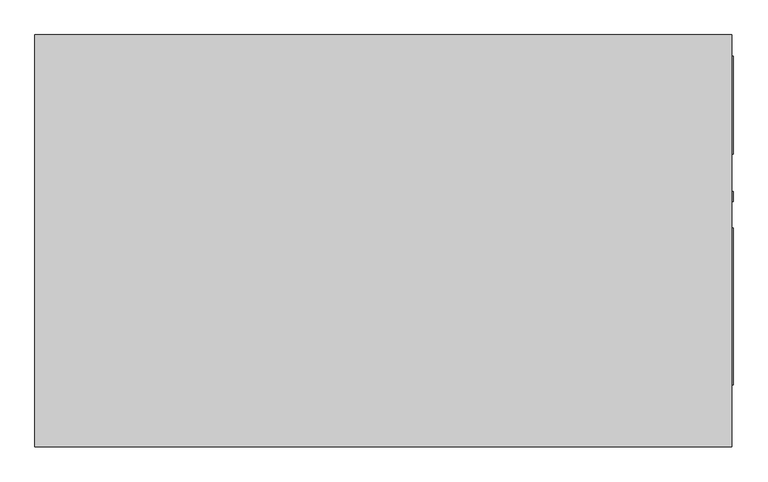
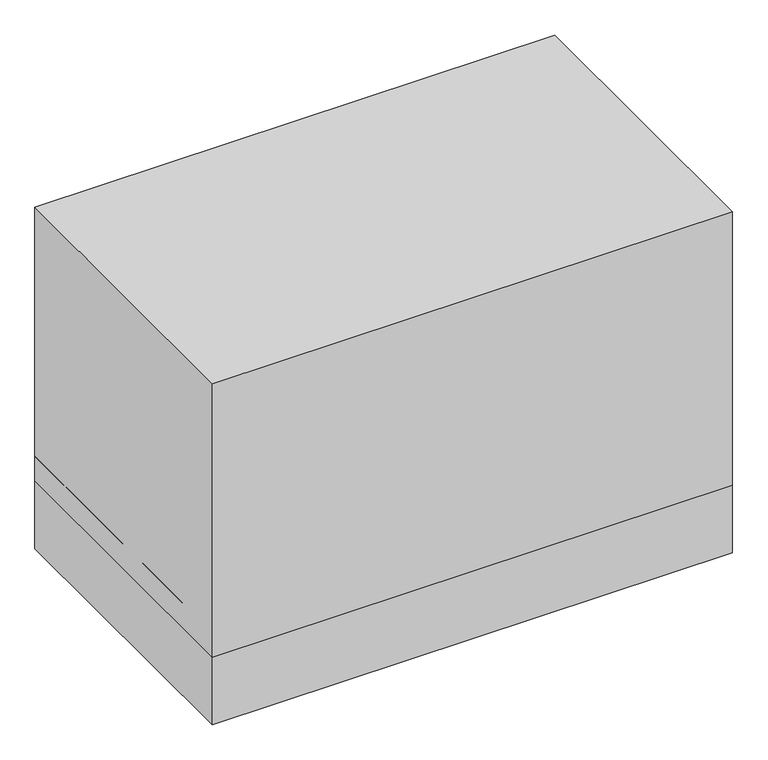
"""IFC4 building model written with IfcOpenShell, lengths in millimetres: proxy geometry, Carrier_48TC_Standard_Efficiency_Gas_Heat_Electric_Cooling_Packaged_Rooftop_Unit_3_to_15_nominal_tons : 6 ton 48TC**07."""

from ifc_helpers import new_model, si_unit, point, frame, frame_2d, origin, origin_with_axes, place, context, project, spatial, polyline, circle_curve, trimmed, segment, composite_curve, outline, extrude, source, transform, mapped, element, save
from ifc_brep_helpers import plane_surface, revolved_surface, advanced_brep


def mechanical_equipment_a9af85ce(model_context):
    return source(origin(), model_context, "Body", "SolidModel", [
        extrude(outline(composite_curve([segment(trimmed(circle_curve(frame_2d((120.65, 438.15)), 13.2953125), [point((107.3546875, 438.15))], [point((133.9453125, 438.15))], False, "CARTESIAN"), True, "CONTINUOUS"), segment(trimmed(circle_curve(frame_2d((120.65, 438.15)), 13.2953125), [point((133.9453125, 438.15))], [point((107.3546875, 438.15))], False, "CARTESIAN"), True, "CONTINUOUS")], self_intersect=False)), frame((944.5625, 0.0, 0.0), z_axis=(1.0, 0.0, 0.0), x_axis=(0.0, 1.0, 0.0)), (0.0, 0.0, 1.0), 3.175),
        advanced_brep(
        [(944.5625, 558.8, 1311.275), (-944.5625, 558.8, 1311.275), (-944.5625, -558.8, 1311.275), (944.5625, -558.8, 1311.275), (944.5625, 558.8, 260.35), (944.5625, -558.8, 260.35), (-944.5625, -558.8, 260.35), (-944.5625, 558.8, 260.35), (858.8375, -400.05, 260.35), (858.8375, 0.0, 260.35), (550.8625, 0.0, 260.35), (550.8625, -400.05, 260.35), (858.8375, 463.55, 260.35), (207.9625, 463.55, 260.35), (207.9625, 187.325, 260.35), (858.8375, 187.325, 260.35), (284.7578125, -88.9, 260.35), (258.1671875, -88.9, 260.35), (-298.45, -247.65, 260.35), (-320.675, -247.65, 260.35), (-295.275, -149.225, 260.35), (-323.85, -149.225, 260.35), (-294.48125, -98.425, 260.35), (-324.64375, -98.425, 260.35), (858.8375, -400.05, 381.0), (550.8625, -400.05, 381.0), (550.8625, 0.0, 381.0), (858.8375, 0.0, 381.0), (858.8375, 463.55, 381.0), (858.8375, 187.325, 381.0), (207.9625, 187.325, 381.0), (207.9625, 463.55, 381.0), (284.7578125, -88.9, 415.925), (258.1671875, -88.9, 415.925), (-298.45, -247.65, 415.925), (-320.675, -247.65, 415.925), (-295.275, -149.225, 415.925), (-323.85, -149.225, 415.925), (-294.48125, -98.425, 415.925), (-324.64375, -98.425, 415.925)],
        [
            (0, 1),
            (1, 2),
            (2, 3),
            (3, 0),
            (4, 5),
            (5, 6),
            (6, 7),
            (7, 4),
            (8, 9),
            (9, 10),
            (10, 11),
            (11, 8),
            (12, 13),
            (13, 14),
            (14, 15),
            (15, 12),
            (16, 17, circle_curve(frame((271.4625, -88.9, 260.35), z_axis=(0.0, 0.0, 1.0), x_axis=(-1.0, 0.0, 0.0)), 13.2953125)),
            (17, 16, circle_curve(frame((271.4625, -88.9, 260.35), z_axis=(0.0, 0.0, 1.0), x_axis=(-1.0, 0.0, 0.0)), 13.2953125)),
            (18, 19, circle_curve(frame((-309.5625, -247.65, 260.35), z_axis=(0.0, 0.0, 1.0), x_axis=(-1.0, 0.0, 0.0)), 11.1125)),
            (19, 18, circle_curve(frame((-309.5625, -247.65, 260.35), z_axis=(0.0, 0.0, 1.0), x_axis=(-1.0, 0.0, 0.0)), 11.1125)),
            (20, 21, circle_curve(frame((-309.5625, -149.225, 260.35), z_axis=(0.0, 0.0, 1.0), x_axis=(-1.0, 0.0, 0.0)), 14.2875)),
            (21, 20, circle_curve(frame((-309.5625, -149.225, 260.35), z_axis=(0.0, 0.0, 1.0), x_axis=(-1.0, 0.0, 0.0)), 14.2875)),
            (22, 23, circle_curve(frame((-309.5625, -98.425, 260.35), z_axis=(0.0, 0.0, 1.0), x_axis=(-1.0, 0.0, 0.0)), 15.08125)),
            (23, 22, circle_curve(frame((-309.5625, -98.425, 260.35), z_axis=(0.0, 0.0, 1.0), x_axis=(-1.0, 0.0, 0.0)), 15.08125)),
            (0, 4),
            (7, 1),
            (6, 2),
            (5, 3),
            (24, 25),
            (25, 26),
            (26, 27),
            (27, 24),
            (27, 9),
            (8, 24),
            (26, 10),
            (25, 11),
            (28, 29),
            (29, 30),
            (30, 31),
            (31, 28),
            (31, 13),
            (12, 28),
            (30, 14),
            (29, 15),
            (32, 33, circle_curve(frame((271.4625, -88.9, 415.925), z_axis=(0.0, 0.0, -1.0), x_axis=(-1.0, 0.0, 0.0)), 13.2953125)),
            (33, 32, circle_curve(frame((271.4625, -88.9, 415.925), z_axis=(0.0, 0.0, -1.0), x_axis=(-1.0, 0.0, 0.0)), 13.2953125)),
            (33, 17),
            (16, 32),
            (34, 35, circle_curve(frame((-309.5625, -247.65, 415.925), z_axis=(0.0, 0.0, -1.0), x_axis=(-1.0, 0.0, 0.0)), 11.1125)),
            (35, 34, circle_curve(frame((-309.5625, -247.65, 415.925), z_axis=(0.0, 0.0, -1.0), x_axis=(-1.0, 0.0, 0.0)), 11.1125)),
            (35, 19),
            (18, 34),
            (36, 37, circle_curve(frame((-309.5625, -149.225, 415.925), z_axis=(0.0, 0.0, -1.0), x_axis=(-1.0, 0.0, 0.0)), 14.2875)),
            (37, 36, circle_curve(frame((-309.5625, -149.225, 415.925), z_axis=(0.0, 0.0, -1.0), x_axis=(-1.0, 0.0, 0.0)), 14.2875)),
            (37, 21),
            (20, 36),
            (38, 39, circle_curve(frame((-309.5625, -98.425, 415.925), z_axis=(0.0, 0.0, -1.0), x_axis=(-1.0, 0.0, 0.0)), 15.08125)),
            (39, 38, circle_curve(frame((-309.5625, -98.425, 415.925), z_axis=(0.0, 0.0, -1.0), x_axis=(-1.0, 0.0, 0.0)), 15.08125)),
            (39, 23),
            (22, 38),
        ],
        [
            plane_surface(frame((-944.5625, 558.8, 1311.275), z_axis=(0.0, 0.0, 1.0), x_axis=(-1.0, 0.0, 0.0))),
            plane_surface(frame((-944.5625, 558.8, 260.35), z_axis=(0.0, 0.0, -1.0), x_axis=(1.0, 0.0, 0.0))),
            plane_surface(frame((944.5625, 558.8, 1311.275), z_axis=(0.0, 1.0, 0.0), x_axis=(0.0, 0.0, -1.0))),
            plane_surface(frame((-944.5625, 558.8, 1311.275), z_axis=(-1.0, 0.0, 0.0), x_axis=(0.0, 0.0, -1.0))),
            plane_surface(frame((-944.5625, -558.8, 1311.275), z_axis=(0.0, -1.0, 0.0), x_axis=(0.0, 0.0, -1.0))),
            plane_surface(frame((944.5625, -558.8, 1311.275), z_axis=(1.0, 0.0, 0.0), x_axis=(0.0, 0.0, -1.0))),
            plane_surface(frame((858.8375, -400.05, 381.0), z_axis=(0.0, 0.0, -1.0), x_axis=(0.0, 1.0, 0.0))),
            plane_surface(frame((858.8375, -400.05, 381.0), z_axis=(-1.0, 0.0, 0.0), x_axis=(0.0, 0.0, -1.0))),
            plane_surface(frame((858.8375, 0.0, 381.0), z_axis=(0.0, -1.0, 0.0), x_axis=(0.0, 0.0, -1.0))),
            plane_surface(frame((550.8625, 0.0, 381.0), z_axis=(1.0, 0.0, 0.0), x_axis=(0.0, 0.0, -1.0))),
            plane_surface(frame((550.8625, -400.05, 381.0), z_axis=(0.0, 1.0, 0.0), x_axis=(0.0, 0.0, -1.0))),
            plane_surface(frame((207.9625, 463.55, 381.0), z_axis=(0.0, 0.0, -1.0), x_axis=(-1.0, 0.0, 0.0))),
            plane_surface(frame((858.8375, 463.55, 381.0), z_axis=(0.0, -1.0, 0.0), x_axis=(0.0, 0.0, -1.0))),
            plane_surface(frame((207.9625, 463.55, 381.0), z_axis=(1.0, 0.0, 0.0), x_axis=(0.0, 0.0, -1.0))),
            plane_surface(frame((207.9625, 187.325, 381.0), z_axis=(0.0, 1.0, 0.0), x_axis=(0.0, 0.0, -1.0))),
            plane_surface(frame((858.8375, 187.325, 381.0), z_axis=(-1.0, 0.0, 0.0), x_axis=(0.0, 0.0, -1.0))),
            plane_surface(frame((258.1671875, -88.9, 415.925), z_axis=(0.0, 0.0, -1.0), x_axis=(0.0, -1.0, 0.0))),
            revolved_surface(polyline([(258.16718749999995, -88.9, 415.925), (258.16718749999995, -88.9, 260.35)]), (271.4625, -88.9, 0.0), (0.0, 0.0, 1.0)),
            plane_surface(frame((-320.675, -247.65, 415.925), z_axis=(0.0, 0.0, -1.0), x_axis=(0.0, -1.0, 0.0))),
            revolved_surface(polyline([(-320.675, -247.65, 415.925), (-320.675, -247.65, 260.35)]), (-309.5625, -247.65, 0.0), (0.0, 0.0, 1.0)),
            plane_surface(frame((-323.85, -149.225, 415.925), z_axis=(0.0, 0.0, -1.0), x_axis=(0.0, -1.0, 0.0))),
            revolved_surface(polyline([(-323.85, -149.225, 415.925), (-323.85, -149.225, 260.35)]), (-309.5625, -149.225, 0.0), (0.0, 0.0, 1.0)),
            plane_surface(frame((-324.64375, -98.425, 415.925), z_axis=(0.0, 0.0, -1.0), x_axis=(0.0, -1.0, 0.0))),
            revolved_surface(polyline([(-324.64375, -98.425, 415.925), (-324.64375, -98.425, 260.35)]), (-309.5625, -98.425, 0.0), (0.0, 0.0, 1.0)),
        ],
        [
            (0, [[1, 2, 3, 4]]),
            (1, [[5, 6, 7, 8], [9, 10, 11, 12], [13, 14, 15, 16], [17, 18], [19, 20], [21, 22], [23, 24]]),
            (2, [[-1, 25, -8, 26]]),
            (3, [[-2, -26, -7, 27]]),
            (4, [[-3, -27, -6, 28]]),
            (5, [[-4, -28, -5, -25]]),
            (6, [[29, 30, 31, 32]]),
            (7, [[-32, 33, -9, 34]]),
            (8, [[-31, 35, -10, -33]]),
            (9, [[-30, 36, -11, -35]]),
            (10, [[-29, -34, -12, -36]]),
            (11, [[37, 38, 39, 40]]),
            (12, [[-40, 41, -13, 42]]),
            (13, [[-39, 43, -14, -41]]),
            (14, [[-38, 44, -15, -43]]),
            (15, [[-37, -42, -16, -44]]),
            (16, [[45, 46]]),
            (17, [[-46, 47, -17, 48]]),
            (17, [[-45, -48, -18, -47]]),
            (18, [[49, 50]]),
            (19, [[-50, 51, -19, 52]]),
            (19, [[-49, -52, -20, -51]]),
            (20, [[53, 54]]),
            (21, [[-54, 55, -21, 56]]),
            (21, [[-53, -56, -22, -55]]),
            (22, [[57, 58]]),
            (23, [[-58, 59, -23, 60]]),
            (23, [[-57, -60, -24, -59]]),
        ],
    ),
        extrude(outline(polyline([(944.5625, 558.8), (944.5625, -558.8), (-944.5625, -558.8), (-944.5625, 558.8), (944.5625, 558.8)]), holes=[polyline([(858.8375, 463.55), (207.9625, 463.55), (207.9625, 187.325), (858.8375, 187.325), (858.8375, 463.55)]), polyline([(858.8375, -400.05), (858.8375, 0.0), (550.8625, 0.0), (550.8625, -400.05), (858.8375, -400.05)]), composite_curve([segment(trimmed(circle_curve(frame_2d((271.4625, -88.9)), 13.2953125), [point((284.7578125, -88.9))], [point((258.1671875, -88.9))], True, "CARTESIAN"), True, "CONTINUOUS"), segment(trimmed(circle_curve(frame_2d((271.4625, -88.9)), 13.2953125), [point((258.1671875, -88.9))], [point((284.7578125, -88.9))], True, "CARTESIAN"), True, "CONTINUOUS")], self_intersect=False), composite_curve([segment(trimmed(circle_curve(frame_2d((-309.5625, -247.65)), 11.1125), [point((-298.45, -247.65))], [point((-320.675, -247.65))], True, "CARTESIAN"), True, "CONTINUOUS"), segment(trimmed(circle_curve(frame_2d((-309.5625, -247.65)), 11.1125), [point((-320.675, -247.65))], [point((-298.45, -247.65))], True, "CARTESIAN"), True, "CONTINUOUS")], self_intersect=False), composite_curve([segment(trimmed(circle_curve(frame_2d((-309.5625, -149.225)), 14.2875), [point((-295.275, -149.225))], [point((-323.85, -149.225))], True, "CARTESIAN"), True, "CONTINUOUS"), segment(trimmed(circle_curve(frame_2d((-309.5625, -149.225)), 14.2875), [point((-323.85, -149.225))], [point((-295.275, -149.225))], True, "CARTESIAN"), True, "CONTINUOUS")], self_intersect=False), composite_curve([segment(trimmed(circle_curve(frame_2d((-309.5625, -98.425)), 15.08125), [point((-294.48125, -98.425))], [point((-324.64375, -98.425))], True, "CARTESIAN"), True, "CONTINUOUS"), segment(trimmed(circle_curve(frame_2d((-309.5625, -98.425)), 15.08125), [point((-324.64375, -98.425))], [point((-294.48125, -98.425))], True, "CARTESIAN"), True, "CONTINUOUS")], self_intersect=False)]), origin_with_axes(), (0.0, 0.0, 1.0), 355.6),
        extrude(outline(polyline([(947.7375, 501.65), (947.7375, 234.95), (944.5625, 234.95), (944.5625, 501.65), (947.7375, 501.65)])), frame((0.0, 0.0, 412.75), z_axis=(0.0, 0.0, 1.0), x_axis=(1.0, 0.0, 0.0)), (0.0, 0.0, 1.0), 638.175),
        extrude(outline(polyline([(947.7375, 34.925), (947.7375, -390.525), (944.5625, -390.525), (944.5625, 34.925), (947.7375, 34.925)])), frame((0.0, 0.0, 415.925), z_axis=(0.0, 0.0, 1.0), x_axis=(1.0, 0.0, 0.0)), (0.0, 0.0, 1.0), 288.925),
    ])


if __name__ == "__main__":
    model = new_model("IFC4")
    model_context = context("Model", 3, world=origin())
    ifc_project = project(units=[si_unit("LENGTHUNIT", "METRE", prefix="MILLI")], contexts=[model_context])
    site = spatial("IfcSite", under=ifc_project)
    building = spatial("IfcBuilding", under=site)
    placement = place(None, origin())
    mechanical_equipment_shape = mechanical_equipment_a9af85ce(model_context)
    element("IfcBuildingElementProxy", 1, Name="Carrier_48TC_Standard_Efficiency_Gas_Heat_Electric_Cooling_Packaged_Rooftop_Unit_3_to_15_nominal_tons : 6 ton 48TC**07", ObjectType="Carrier_48TC_Standard_Efficiency_Gas_Heat_Electric_Cooling_Packaged_Rooftop_Unit_3_to_15_nominal_tons : 6 ton 48TC**07", at=placement, inside=building, context=model_context, shape_type="MappedRepresentation", body=[
        mapped(mechanical_equipment_shape, transform((0.0, 0.0, 0.0), x_axis=(1.0, 0.0, 0.0), y_axis=(0.0, 1.0, 0.0), z_axis=(0.0, 0.0, 1.0))),
    ])
    save(model, "model.ifc")

# Revit data of these elements
# Type "Carrier_48TC_Standard_Efficiency_Gas_Heat_Electric_Cooling_Packaged_Rooftop_Unit_3_to_15_nominal_tons : 6 ton 48TC**07"
#   URL = "www.Carrier.com"
#   Model = "48TC"
#   Manufacturer = "Carrier"
#   Disclaimer = "Manufacturer reserves the right to change, at any time, specifications and designs without notice and without obligation.  Please verify critical parameters with local Carrier commercial sales office."
#   knockout thickness = 0' - 0 1/16"
#   Voltage = 0 V
#   Version = 1
#   TTBY3 = 1' - 0 1/4"
#   TTBY2 = 1' - 4 1/8"
#   TTBY1 = 1' - 6 1/8"
#   TTBX = 2' - 1"
#   TTBPowerR = 0' - 0 9/16"
#   TTBGasR = 0' - 0 19/32"
#   SSSZ = 0' - 6 1/8"
#   SSSY = 0' - 6 5/8"
#   SSSW = 1' - 4 3/4"
#   SSSH = 0' - 11 3/8"
#   SSRZ = 0' - 6"
#   SSRY = 0' - 2 1/4"
#   SSRW = 0' - 10 1/2"
#   SSRH = 2' - 1 1/8"
#   SEER = 0
#   Right clearance = 3' - 0"
#   PWRZ = 1' - 3 3/4"
#   PWRY = 0' - 4 5/8"
#   PWRR = 0' - 1 1/4"
#   ODF2X = 3' - 6"
#   ODF1Y = 1' - 2"
#   ODF1X = 1' - 2"
#   ODF1R = 1' - 1"
#   MOCP = 0 A
#   MCA = 0 A
#   Left clearance = 4' - 0"
#   IEER = 11.2
#   Front clearance = 4' - 0"
#   Fan Z = 4' - 3 5/8"
#   Width = 3' - 8"
#   Length = 6' - 2 3/8"
#   Height = 3' - 5 3/8"
#   EER = 11
#   DSSY = 0' - 6 1/4"
#   DSSX = 0' - 3 3/8"
#   DSSW = 1' - 0 1/8"
#   DSSH = 1' - 5 3/4"
#   DSRY = 0' - 3 3/4"
#   DSRX = 0' - 3 3/8"
#   DSRW = 2' - 1 5/8"
#   DSRH = 0' - 10 7/8"
#   DRNZ = 0' - 7"
#   DRNY = 2' - 2 3/4"
#   DRNR = 0' - 0 67/128"
#   Curb Z = 1' - 2"
#   CFM (nominal) = 0 CFM
#   Back clearance = 3' - 0"
#   Alt Condensate Drain = 0' - 0 67/128"
#   AccypwrR = 0' - 0 7/16"
#   ACY = 1' - 6 1/2"
#   ACX = 2' - 2 1/2"
#   Gas [instance default] = yes
#   Fan 2 on = no
#   Curb_1SLAB_2ROOFCURB_3SNOWCURB = 2
#   Fan 3 on = no
#   Unit material = SINGLE-PACKAGED ROOFTOP UNITS
#   Curb material = Curb paint
# Element 1 (IfcBuildingElementProxy, "Carrier_48TC_Standard_Efficiency_Gas_Heat_Electric_Cooling_Packaged_Rooftop_Unit_3_to_15_nominal_tons : 6 ton 48TC**07")
#   Materials on its faces: "SINGLE-PACKAGED ROOFTOP UNITS", "Curb paint", "Mech"
# Materials
#   "SINGLE-PACKAGED ROOFTOP UNITS": class "Miscellaneous", colour RGB 201 201 201, transparency 0, Cost = 0
#   "Curb paint": class "Miscellaneous", colour RGB 189 187 185, transparency 0
#   "Mech": class "Miscellaneous", colour RGB 235 237 235, transparency 0, Cost = 0
